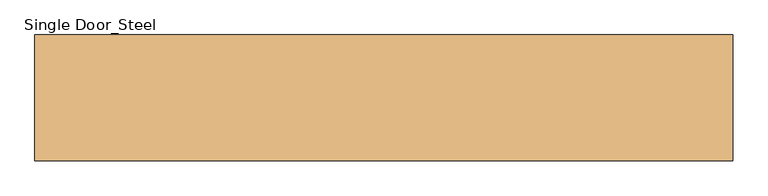
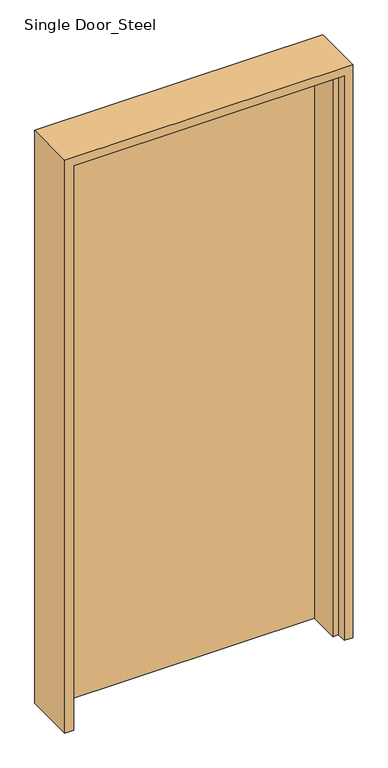
"""IFC4 building model written with IfcOpenShell, lengths in millimetres: door geometry, Single Door_Steel : H_DR_AR_B12_Single Door_Steel_W1000xH2100_0.5Hr."""

from ifc_helpers import new_model, si_unit, origin, origin_with_axes, place, context, project, spatial, polyline, outline, extrude, faceted_brep, source, transform, mapped, element, save


def single_door_steel_d0b2540c(model_context):
    return source(origin(), model_context, "Body", "SolidModel", [
        extrude(outline(polyline([(470.0, 90.0), (470.0, 55.0), (-470.0, 55.0), (-470.0, 90.0), (470.0, 90.0)])), origin_with_axes(), (0.0, 0.0, 1.0), 2070.0),
        faceted_brep([(470.0, 90.0, 0.0), (500.0, 90.0, 0.0), (500.0, -90.0, 0.0), (470.0, -90.0, 0.0), (470.0, -55.0, 0.0), (450.0, -55.0, 0.0), (450.0, 55.0, 0.0), (470.0, 55.0, 0.0), (470.0, 90.0, 2070.0), (-470.0, 90.0, 2070.0), (-470.0, 90.0, 0.0), (-500.0, 90.0, 0.0), (-500.0, 90.0, 2100.0), (500.0, 90.0, 2100.0), (500.0, -90.0, 2100.0), (-500.0, -90.0, 2100.0), (-500.0, -90.0, 0.0), (-470.0, -90.0, 0.0), (-470.0, -90.0, 2070.0), (470.0, -90.0, 2070.0), (470.0, -55.0, 2070.0), (-470.0, -55.0, 2070.0), (-470.0, -55.0, 0.0), (-450.0, -55.0, 0.0), (-450.0, -55.0, 2050.0), (450.0, -55.0, 2050.0), (450.0, 55.0, 2050.0), (-450.0, 55.0, 2050.0), (-450.0, 55.0, 0.0), (-470.0, 55.0, 0.0), (-470.0, 55.0, 2070.0), (470.0, 55.0, 2070.0)], [[[0, 1, 2, 3, 4, 5, 6, 7]], [[1, 0, 8, 9, 10, 11, 12, 13]], [[2, 1, 13, 14]], [[3, 2, 14, 15, 16, 17, 18, 19]], [[4, 3, 19, 20]], [[5, 4, 20, 21, 22, 23, 24, 25]], [[6, 5, 25, 26]], [[7, 6, 26, 27, 28, 29, 30, 31]], [[0, 7, 31, 8]], [[9, 30, 29, 10]], [[10, 29, 28, 23, 22, 17, 16, 11]], [[15, 12, 11, 16]], [[21, 18, 17, 22]], [[27, 24, 23, 28]], [[14, 13, 12, 15]], [[20, 19, 18, 21]], [[26, 25, 24, 27]], [[8, 31, 30, 9]]]),
    ])


if __name__ == "__main__":
    model = new_model("IFC4")
    model_context = context("Model", 3, world=origin())
    ifc_project = project(units=[si_unit("LENGTHUNIT", "METRE", prefix="MILLI")], contexts=[model_context])
    site = spatial("IfcSite", under=ifc_project)
    building = spatial("IfcBuilding", under=site)
    placement = place(None, origin())
    single_door_steel_shape = single_door_steel_d0b2540c(model_context)
    element("IfcDoor", 1, ObjectType="Single Door_Steel : H_DR_AR_B12_Single Door_Steel_W1000xH2100_0.5Hr", at=placement, inside=building, context=model_context, shape_type="MappedRepresentation", body=[
        mapped(single_door_steel_shape, transform((0.0, 0.0, 0.0), x_axis=(1.0, 0.0, 0.0), y_axis=(0.0, 1.0, 0.0), z_axis=(0.0, 0.0, 1.0))),
    ])
    save(model, "model.ifc")

# Revit data of these elements
# Type "Single Door_Steel : H_DR_AR_B12_Single Door_Steel_W1000xH2100_0.5Hr"
#   Type Mark = "SD"
#   Analytic Construction = "<None>"
#   프레임 투영 외부. = 25 mm
#   프레임 투영 내부. = 25 mm
#   프레임 폭 = 75 mm
#   Height = 2100 mm
#   Width = 1000 mm
#   Define Thermal Properties by = 1
#   문 패널 = none
#   문 프레임 = none
#   Function = (empty or 0)
#   Wall Closure = (empty or 0)
